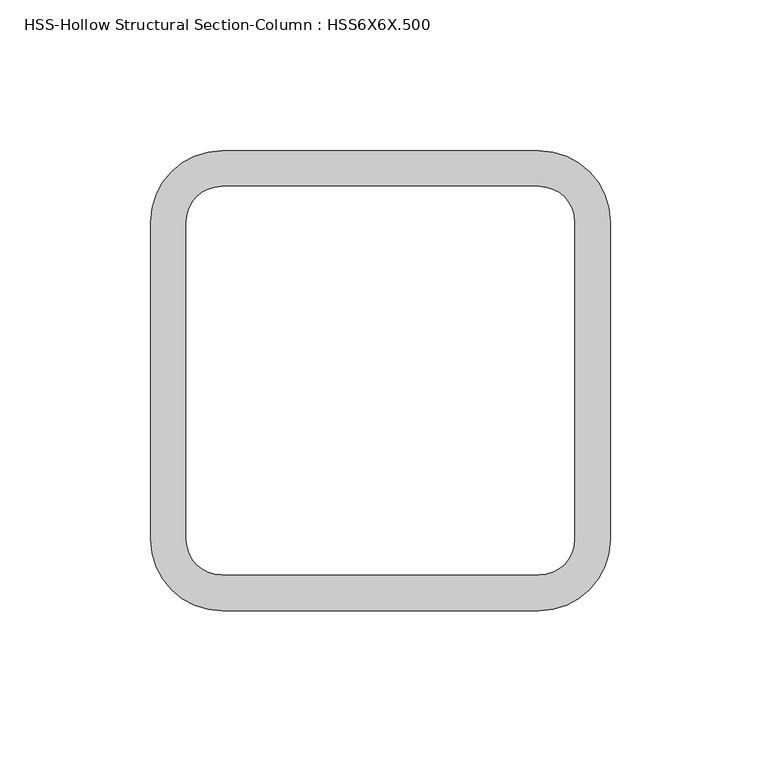
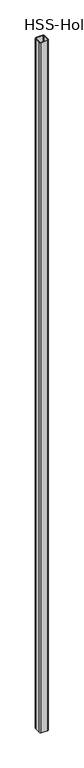
"""IFC4 building model written with IfcOpenShell, lengths in millimetres: column geometry, HSS-Hollow Structural Section-Column : HSS6X6X.500."""

from ifc_helpers import new_model, si_unit, point, frame, frame_2d, origin, place, context, project, spatial, polyline, circle_curve, trimmed, segment, composite_curve, outline, extrude, source, transform, mapped, element, save


def hss_hollow_structural_section_column_hss6x6x_500_4d0a40ad(model_context):
    return source(origin(), model_context, "Body", "SweptSolid", [
        extrude(outline(composite_curve([segment(trimmed(circle_curve(frame_2d((52.5859375, 52.5859375)), 23.6140625), [point((52.5859375, 76.2))], [point((76.2, 52.5859375))], False, "CARTESIAN"), True, "CONTINUOUS"), segment(polyline([(76.2, 52.5859375), (76.2, -52.5859375)]), True, "CONTINUOUS"), segment(trimmed(circle_curve(frame_2d((52.5859375, -52.5859375)), 23.6140625), [point((76.2, -52.5859375))], [point((52.5859375, -76.2))], False, "CARTESIAN"), True, "CONTINUOUS"), segment(polyline([(52.5859375, -76.2), (-52.5859375, -76.2)]), True, "CONTINUOUS"), segment(trimmed(circle_curve(frame_2d((-52.5859375, -52.5859375)), 23.6140625), [point((-52.5859375, -76.2))], [point((-76.2, -52.5859375))], False, "CARTESIAN"), True, "CONTINUOUS"), segment(polyline([(-76.2, -52.5859375), (-76.2, 52.5859375)]), True, "CONTINUOUS"), segment(trimmed(circle_curve(frame_2d((-52.5859375, 52.5859375)), 23.6140625), [point((-76.2, 52.5859375))], [point((-52.5859375, 76.2))], False, "CARTESIAN"), True, "CONTINUOUS"), segment(polyline([(-52.5859375, 76.2), (52.5859375, 76.2)]), True, "CONTINUOUS")], self_intersect=False), holes=[composite_curve([segment(polyline([(52.5859375, 64.3929688), (-52.5859375, 64.3929688)]), True, "CONTINUOUS"), segment(trimmed(circle_curve(frame_2d((-52.5859375, 52.5859375)), 11.8070313), [point((-52.5859375, 64.3929688))], [point((-64.3929688, 52.5859375))], True, "CARTESIAN"), True, "CONTINUOUS"), segment(polyline([(-64.3929688, 52.5859375), (-64.3929688, -52.5859375)]), True, "CONTINUOUS"), segment(trimmed(circle_curve(frame_2d((-52.5859375, -52.5859375)), 11.8070313), [point((-64.3929688, -52.5859375))], [point((-52.5859375, -64.3929687))], True, "CARTESIAN"), True, "CONTINUOUS"), segment(polyline([(-52.5859375, -64.3929687), (52.5859375, -64.3929687)]), True, "CONTINUOUS"), segment(trimmed(circle_curve(frame_2d((52.5859375, -52.5859375)), 11.8070312), [point((52.5859375, -64.3929687))], [point((64.3929687, -52.5859375))], True, "CARTESIAN"), True, "CONTINUOUS"), segment(polyline([(64.3929687, -52.5859375), (64.3929687, 52.5859375)]), True, "CONTINUOUS"), segment(trimmed(circle_curve(frame_2d((52.5859375, 52.5859375)), 11.8070312), [point((64.3929687, 52.5859375))], [point((52.5859375, 64.3929688))], True, "CARTESIAN"), True, "CONTINUOUS")], self_intersect=False)]), frame((0.0, 0.0, -609.6), z_axis=(0.0, 0.0, 1.0), x_axis=(1.0, 0.0, 0.0)), (0.0, 0.0, 1.0), 12484.1),
    ])


if __name__ == "__main__":
    model = new_model("IFC4")
    model_context = context("Model", 3, world=origin())
    ifc_project = project(units=[si_unit("LENGTHUNIT", "METRE", prefix="MILLI")], contexts=[model_context])
    site = spatial("IfcSite", under=ifc_project)
    building = spatial("IfcBuilding", under=site)
    placement = place(None, origin())
    hss_hollow_structural_section_column_hss6x6x_500_shape = hss_hollow_structural_section_column_hss6x6x_500_4d0a40ad(model_context)
    element("IfcColumn", 1, ObjectType="HSS-Hollow Structural Section-Column : HSS6X6X.500", at=placement, inside=building, context=model_context, shape_type="MappedRepresentation", body=[
        mapped(hss_hollow_structural_section_column_hss6x6x_500_shape, transform((0.0, 0.0, 0.0), x_axis=(1.0, 0.0, 0.0), y_axis=(0.0, 1.0, 0.0), z_axis=(0.0, 0.0, 1.0))),
    ])
    save(model, "model.ifc")

# Revit data of these elements
# Type "HSS-Hollow Structural Section-Column : HSS6X6X.500"
#   Assembly Code = "B10"
#   Shape = "Square"
#   W = 35.1
#   Ht = 0' - 6"
#   b = 0' - 6"
#   kr = 0' - 0 119/128"
#   t = 0' - 0 119/256"
#   A = 0.07 SF
#   Structural Material [instance default] = Steel ASTM A500, Grade B, Rectangular and Square
# Element 1 (IfcColumn, "HSS-Hollow Structural Section-Column : HSS6X6X.500")
#   Materials on its faces: "Steel ASTM A500, Grade B, Rectangular and Square"
# Materials
#   "Steel ASTM A500, Grade B, Rectangular and Square": class "Metal", colour RGB 199 199 199, transparency 0, Description = "Carbon steel", Cost = 0
